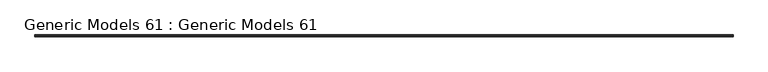
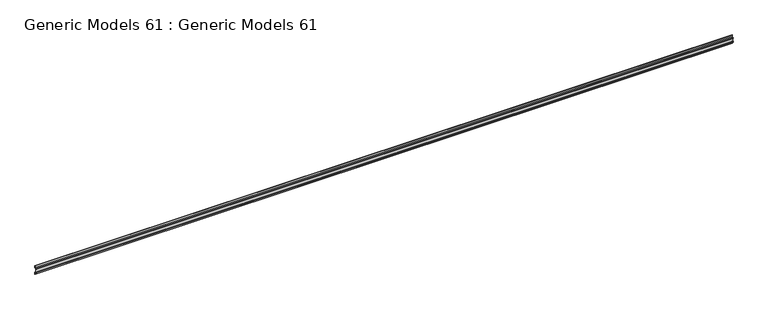
"""IFC4 building model written with IfcOpenShell, lengths in millimetres: proxy geometry, Generic Models 61 : Generic Models 61."""

from ifc_helpers import new_model, si_unit, point, frame, frame_2d, origin, place, context, project, spatial, polyline, circle_curve, trimmed, segment, composite_curve, outline, extrude, source, transform, mapped, element, save


def generic_models_61_generic_models_61_a33eec7a(model_context):
    return source(origin(), model_context, "Body", "SweptSolid", [
        extrude(outline(composite_curve([segment(polyline([(25521.3031612, 266031.6940809), (25512.0590269, 266033.7329782)]), True, "CONTINUOUS"), segment(trimmed(circle_curve(frame_2d((25512.5719112, 266036.0583386)), 2.38125), [point((25512.0590269, 266033.7329782))], [point((25510.9844112, 266037.8332176))], False, "CARTESIAN"), True, "CONTINUOUS"), segment(trimmed(circle_curve(frame_2d((25509.3969112, 266039.6080965)), 2.38125), [point((25510.9844112, 266037.8332176))], [point((25511.7781612, 266039.6080965))], True, "CARTESIAN"), True, "CONTINUOUS"), segment(polyline([(25511.7781612, 266039.6080965), (25511.7781612, 266060.2294035)]), True, "CONTINUOUS"), segment(trimmed(circle_curve(frame_2d((25509.3969112, 266060.2294035)), 2.38125), [point((25511.7781612, 266060.2294035))], [point((25510.9844112, 266062.0042824))], True, "CARTESIAN"), True, "CONTINUOUS"), segment(trimmed(circle_curve(frame_2d((25512.5719112, 266063.7791614)), 2.38125), [point((25510.9844112, 266062.0042824))], [point((25512.0590269, 266066.1045218))], False, "CARTESIAN"), True, "CONTINUOUS"), segment(polyline([(25512.0590269, 266066.1045218), (25521.3031612, 266068.1434191), (25521.3031612, 266081.66875), (25522.8906612, 266081.66875), (25522.8906612, 266066.8679047), (25512.4009498, 266064.5542815)]), True, "CONTINUOUS"), segment(trimmed(circle_curve(frame_2d((25512.5719112, 266063.7791614)), 0.79375), [point((25512.4009498, 266064.5542815))], [point((25512.0427445, 266063.1875351))], True, "CARTESIAN"), True, "CONTINUOUS"), segment(trimmed(circle_curve(frame_2d((25509.3969112, 266060.2294035)), 3.96875), [point((25512.0427445, 266063.1875351))], [point((25513.3656612, 266060.2294035))], False, "CARTESIAN"), True, "CONTINUOUS"), segment(polyline([(25513.3656612, 266060.2294035), (25513.3656612, 266039.6080965)]), True, "CONTINUOUS"), segment(trimmed(circle_curve(frame_2d((25509.3969112, 266039.6080965)), 3.96875), [point((25513.3656612, 266039.6080965))], [point((25512.0427445, 266036.6499649))], False, "CARTESIAN"), True, "CONTINUOUS"), segment(trimmed(circle_curve(frame_2d((25512.5719112, 266036.0583386)), 0.79375), [point((25512.0427445, 266036.6499649))], [point((25512.4009498, 266035.2832185))], True, "CARTESIAN"), True, "CONTINUOUS"), segment(polyline([(25512.4009498, 266035.2832185), (25522.8906612, 266032.9695953), (25522.8906612, 266018.16875), (25521.3031612, 266018.16875), (25521.3031612, 266031.6940809)]), True, "CONTINUOUS")], self_intersect=False)), frame((27130.3715778, 0.0, 0.0), z_axis=(1.0, 0.0, 0.0), x_axis=(0.0, 1.0, 0.0)), (0.0, 0.0, 1.0), 5065.7125),
    ])


if __name__ == "__main__":
    model = new_model("IFC4")
    model_context = context("Model", 3, world=origin())
    ifc_project = project(units=[si_unit("LENGTHUNIT", "METRE", prefix="MILLI")], contexts=[model_context])
    site = spatial("IfcSite", under=ifc_project)
    building = spatial("IfcBuilding", under=site)
    placement = place(None, origin())
    generic_models_61_generic_models_61_shape = generic_models_61_generic_models_61_a33eec7a(model_context)
    element("IfcBuildingElementProxy", 1, Name="Generic Models 61 : Generic Models 61", ObjectType="Generic Models 61 : Generic Models 61", at=placement, inside=building, context=model_context, shape_type="MappedRepresentation", body=[
        mapped(generic_models_61_generic_models_61_shape, transform((0.0, 0.0, 0.0), x_axis=(1.0, 0.0, 0.0), y_axis=(0.0, 1.0, 0.0), z_axis=(0.0, 0.0, 1.0))),
    ])
    save(model, "model.ifc")

# Revit data of these elements
# Element 1 (IfcBuildingElementProxy, "Generic Models 61 : Generic Models 61")
#   Materials on its faces: "1/2\" DEEP GALV. HORTZ. HAT CHANNEL @ XX O.C."
# Materials
#   "1/2\" DEEP GALV. HORTZ. HAT CHANNEL @ XX O.C.": class "Generic", colour RGB 212 212 212, transparency 0, Cost = 0
